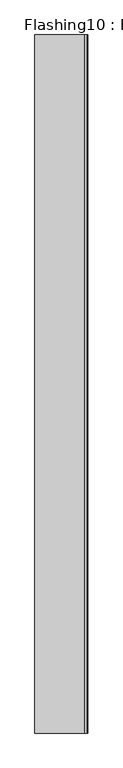
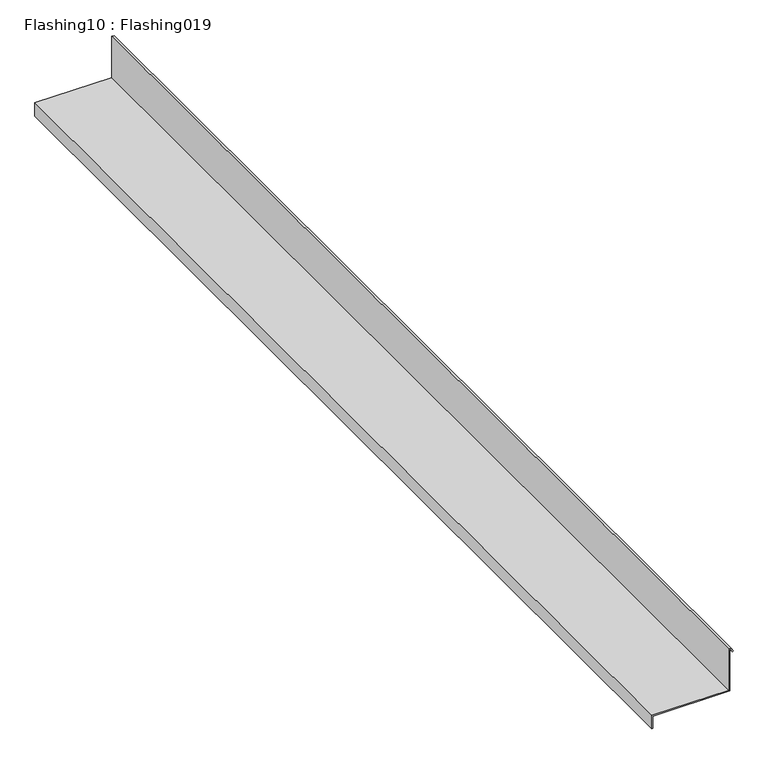
"""IFC4 building model written with IfcOpenShell, lengths in millimetres: proxy geometry, Flashing10 : Flashing019."""

from ifc_helpers import new_model, si_unit, frame, origin, place, context, project, spatial, polyline, outline, extrude, source, transform, mapped, element, save


def flashing10_flashing019_9dc0ec64(model_context):
    return source(origin(), model_context, "Body", "SweptSolid", [
        extrude(outline(polyline([(40784.7382813, 16649.96875), (40784.7382813, 16645.2851562), (40703.2466161, 16645.2851562), (40703.2466161, 16501.84375), (40677.1179688, 16501.84375), (40677.1179688, 16503.84375), (40701.2466161, 16503.84375), (40701.2466161, 16647.2851563), (40782.7382813, 16647.2851563), (40782.7382813, 16648.7903893), (40776.8666698, 16652.0435345), (40777.8359375, 16653.7929687), (40784.7382813, 16649.96875)])), frame((0.0, 7982.1449366, 0.0), z_axis=(0.0, 1.0, 0.0), x_axis=(0.0, 0.0, 1.0)), (0.0, 0.0, 1.0), 2000.0),
    ])


if __name__ == "__main__":
    model = new_model("IFC4")
    model_context = context("Model", 3, world=origin())
    ifc_project = project(units=[si_unit("LENGTHUNIT", "METRE", prefix="MILLI")], contexts=[model_context])
    site = spatial("IfcSite", under=ifc_project)
    building = spatial("IfcBuilding", under=site)
    placement = place(None, origin())
    flashing10_flashing019_shape = flashing10_flashing019_9dc0ec64(model_context)
    element("IfcBuildingElementProxy", 1, Name="Flashing10 : Flashing019", ObjectType="Flashing10 : Flashing019", at=placement, inside=building, context=model_context, shape_type="MappedRepresentation", body=[
        mapped(flashing10_flashing019_shape, transform((0.0, 0.0, 0.0), x_axis=(1.0, 0.0, 0.0), y_axis=(0.0, 1.0, 0.0), z_axis=(0.0, 0.0, 1.0))),
    ])
    save(model, "model.ifc")

# Revit data of these elements
# Type "Flashing10 : Flashing019"
#   NameOverride = "Flashing019"
# Element 1 (IfcBuildingElementProxy, "Flashing10 : Flashing019")
#   Materials on its faces: "BRAKE METAL FLASHING TO MATCH STOREFRONT"
# Materials
#   "BRAKE METAL FLASHING TO MATCH STOREFRONT": class "Unassigned", colour RGB 128 128 128, transparency 0, Cost = 0
